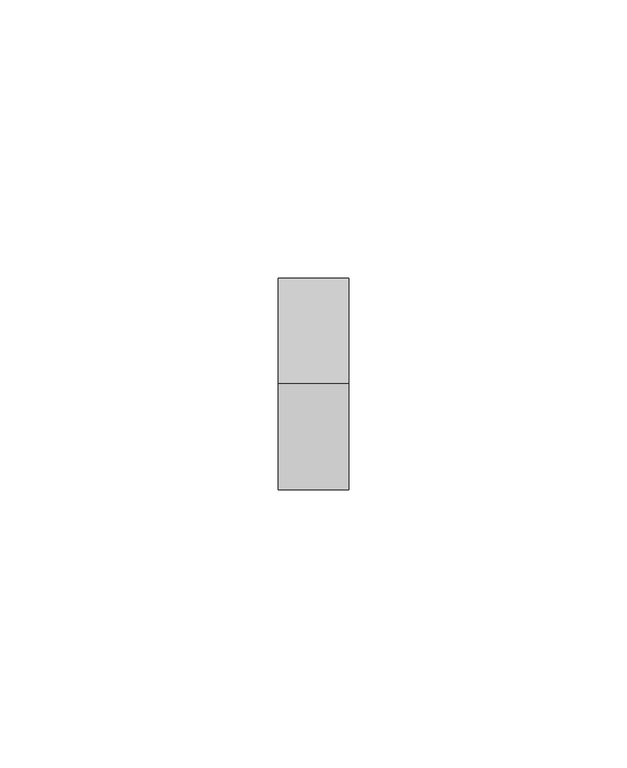
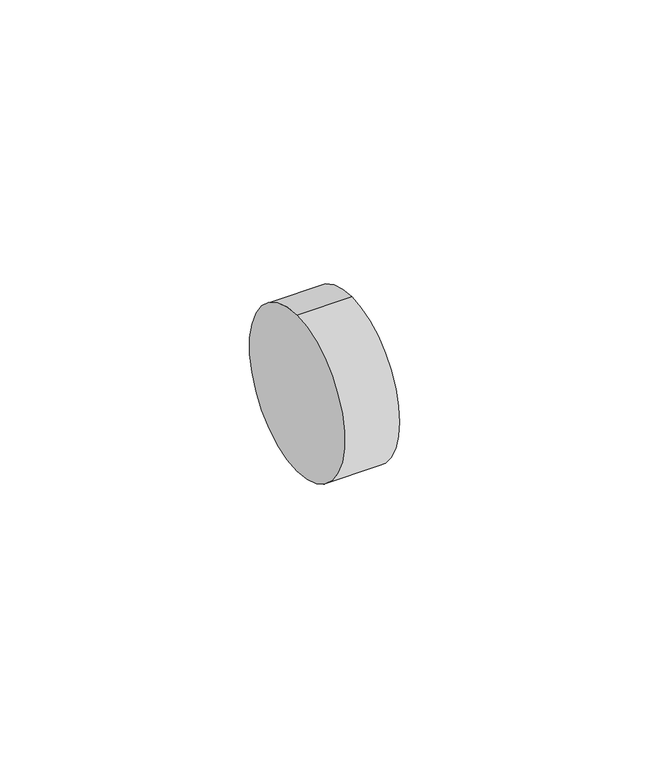
"""IFC4 building model written with IfcOpenShell, lengths in millimetres: proxy geometry, Bolt25:Bolt002:304700 : Bolt25:Bolt002:304700."""

from ifc_helpers import new_model, si_unit, point, frame, frame_2d, origin, place, context, project, spatial, circle_curve, trimmed, segment, composite_curve, outline, extrude, source, transform, mapped, element, save


def generic_models_7e92fd52(model_context):
    return source(origin(), model_context, "Body", "SweptSolid", [
        extrude(outline(composite_curve([segment(trimmed(circle_curve(frame_2d((2174.9207483, 39910.0063132)), 19.05), [point((2174.9207483, 39929.0563132))], [point((2174.9207483, 39890.9563132))], False, "CARTESIAN"), True, "CONTINUOUS"), segment(trimmed(circle_curve(frame_2d((2174.9207483, 39910.0063132)), 19.05), [point((2174.9207483, 39890.9563132))], [point((2174.9207483, 39929.0563132))], False, "CARTESIAN"), True, "CONTINUOUS")], self_intersect=False)), frame((15074.8475949, 0.0, 0.0), z_axis=(1.0, 0.0, 0.0), x_axis=(0.0, 1.0, 0.0)), (0.0, 0.0, 1.0), 12.7),
    ])


if __name__ == "__main__":
    model = new_model("IFC4")
    model_context = context("Model", 3, world=origin())
    ifc_project = project(units=[si_unit("LENGTHUNIT", "METRE", prefix="MILLI")], contexts=[model_context])
    site = spatial("IfcSite", under=ifc_project)
    building = spatial("IfcBuilding", under=site)
    placement = place(None, origin())
    generic_models_shape = generic_models_7e92fd52(model_context)
    element("IfcBuildingElementProxy", 1, Name="Bolt25:Bolt002:304700 : Bolt25:Bolt002:304700", ObjectType="Bolt25:Bolt002:304700 : Bolt25:Bolt002:304700", at=placement, inside=building, context=model_context, shape_type="MappedRepresentation", body=[
        mapped(generic_models_shape, transform((0.0, 0.0, 0.0), x_axis=(1.0, 0.0, 0.0), y_axis=(0.0, 1.0, 0.0), z_axis=(0.0, 0.0, 1.0))),
    ])
    save(model, "model.ifc")

# Revit data of these elements
# Type "Bolt25:Bolt002:304700 : Bolt25:Bolt002:304700"
#   NameOverride = "Bolt25:Bolt002:304700"
#   ObjectTypeOverride = "Bolt25:Bolt002"
#   Reference = "Bolt002"
#   Category = "Generic Models"
#   Tag = "304700"
# Element 1 (IfcBuildingElementProxy, "Bolt25:Bolt002:304700 : Bolt25:Bolt002:304700")
#   Materials on its faces: "TUBE STEEL STRINGER WELDED TO ANCHORED STEEL PLATE - SEE STRUCT DWGS"
# Materials
#   "TUBE STEEL STRINGER WELDED TO ANCHORED STEEL PLATE - SEE STRUCT DWGS": class "Unassigned", colour RGB 128 128 128, transparency 0, Cost = 0
